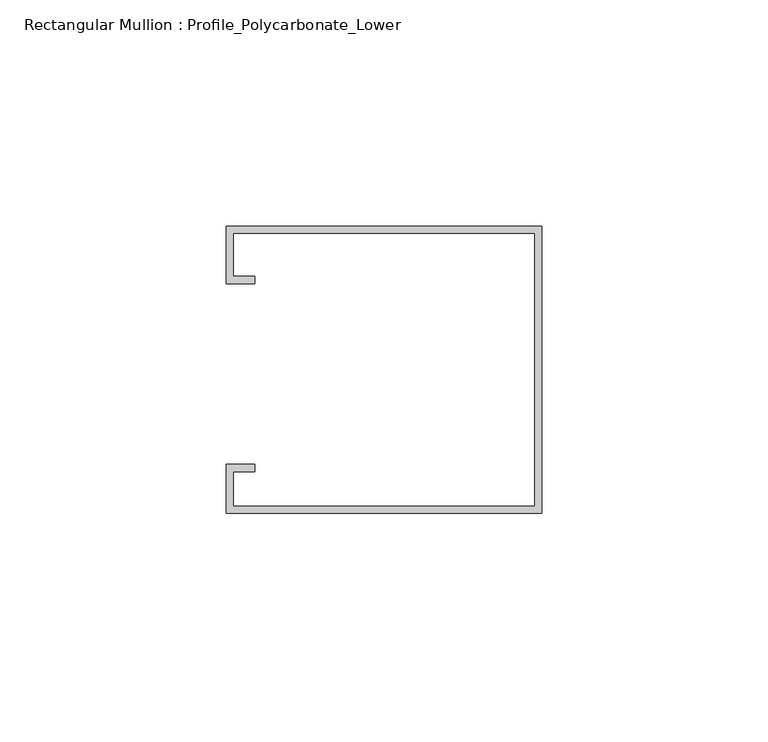
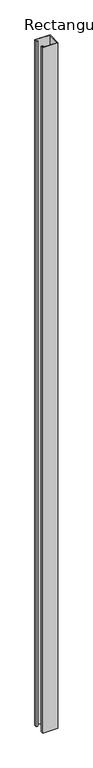
"""IFC4 building model written with IfcOpenShell, lengths in millimetres: member geometry, Rectangular Mullion : Profile_Polycarbonate_Lower."""

from ifc_helpers import new_model, si_unit, frame, origin, place, context, project, spatial, polyline, outline, extrude, source, transform, mapped, element, save


def rectangular_mullion_profile_polycarbonate_lower_dbac95dc(model_context):
    return source(origin(), model_context, "Body", "SweptSolid", [
        extrude(outline(polyline([(0.0, 32.7), (0.0, -30.8), (-69.85, -30.8), (-69.85, -20.0), (-63.5, -20.0), (-63.5, -21.5875), (-68.2625, -21.5875), (-68.2625, -29.2125), (-1.5875, -29.2125), (-1.5875, 31.1125), (-68.2625, 31.1125), (-68.2625, 21.5875), (-63.5, 21.5875), (-63.5, 20.0), (-69.85, 20.0), (-69.85, 32.7), (0.0, 32.7)])), frame((0.0, 0.0, -3351.2125), z_axis=(0.0, 0.0, 1.0), x_axis=(1.0, 0.0, 0.0)), (0.0, 0.0, 1.0), 3351.2125),
    ])


if __name__ == "__main__":
    model = new_model("IFC4")
    model_context = context("Model", 3, world=origin())
    ifc_project = project(units=[si_unit("LENGTHUNIT", "METRE", prefix="MILLI")], contexts=[model_context])
    site = spatial("IfcSite", under=ifc_project)
    building = spatial("IfcBuilding", under=site)
    placement = place(None, origin())
    rectangular_mullion_profile_polycarbonate_lower_shape = rectangular_mullion_profile_polycarbonate_lower_dbac95dc(model_context)
    element("IfcMember", 1, ObjectType="Rectangular Mullion : Profile_Polycarbonate_Lower", at=placement, inside=building, context=model_context, shape_type="MappedRepresentation", body=[
        mapped(rectangular_mullion_profile_polycarbonate_lower_shape, transform((0.0, 0.0, 0.0), x_axis=(1.0, 0.0, 0.0), y_axis=(0.0, 1.0, 0.0), z_axis=(0.0, 0.0, 1.0))),
    ])
    save(model, "model.ifc")

# Revit data of these elements
# Type "Rectangular Mullion : Profile_Polycarbonate_Lower"
#   built-in parameter 1007322 = 0.208333 (stored number, unit not read)
#   built-in parameter 1007321 = 0 (stored number, unit not read)
#   built-in parameter 1007320 = 0.00520833 (stored number, unit not read)
# Element 1 (IfcMember, "Rectangular Mullion : Profile_Polycarbonate_Lower")
#   Materials on its faces: "ALUMINUM PROFILE AT POLYCARBONATE PANEL"
# Materials
#   "ALUMINUM PROFILE AT POLYCARBONATE PANEL": class "Metal", colour RGB 244 244 244, transparency 0, Description = "Aluminum 6061", Cost = 0
